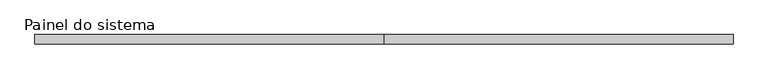
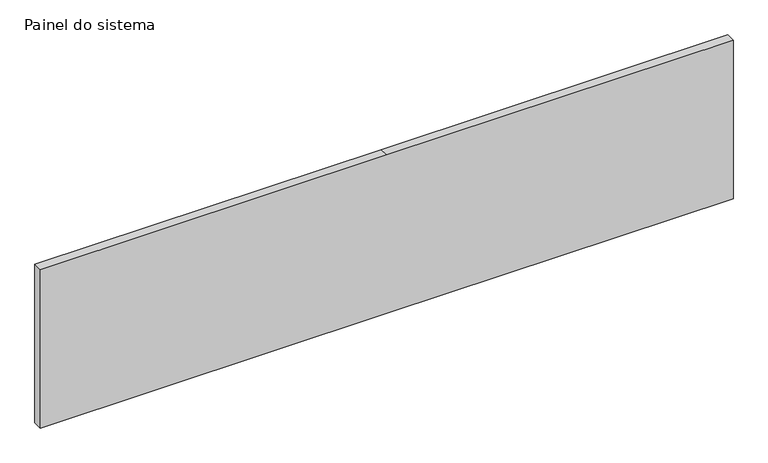
"""IFC4 building model written with IfcOpenShell, lengths in millimetres: plate geometry, Painel do sistema : Envidraçado."""

from ifc_helpers import new_model, si_unit, frame, origin, place, context, project, spatial, polyline, outline, extrude, source, transform, mapped, element, save


def painel_do_sistema_b648e332(model_context):
    return source(origin(), model_context, "Body", "SweptSolid", [
        extrude(outline(polyline([(0.0, -931.0166666), (0.0, 0.0), (0.0, 931.0166666), (450.0, 931.0166666), (450.0, 0.0), (450.0, -931.0166666), (0.0, -931.0166666)])), frame((0.0, 24.5, 0.0), z_axis=(0.0, 1.0, 0.0), x_axis=(0.0, 0.0, 1.0)), (0.0, 0.0, 1.0), 25.0),
    ])


if __name__ == "__main__":
    model = new_model("IFC4")
    model_context = context("Model", 3, world=origin())
    ifc_project = project(units=[si_unit("LENGTHUNIT", "METRE", prefix="MILLI")], contexts=[model_context])
    site = spatial("IfcSite", under=ifc_project)
    building = spatial("IfcBuilding", under=site)
    placement = place(None, origin())
    painel_do_sistema_shape = painel_do_sistema_b648e332(model_context)
    element("IfcPlate", 1, ObjectType="Painel do sistema : Envidraçado", at=placement, inside=building, context=model_context, shape_type="MappedRepresentation", body=[
        mapped(painel_do_sistema_shape, transform((0.0, 0.0, 0.0), x_axis=(1.0, 0.0, 0.0), y_axis=(0.0, 1.0, 0.0), z_axis=(0.0, 0.0, 1.0))),
    ])
    save(model, "model.ifc")

# Revit data of these elements
# Type "Painel do sistema : Envidraçado"
#   Construction Type Id = "GSP4R"
#   Analytic Construction = "Vidraça única Pilkington 1/8 pol"
#   Visual Light Transmittance = 0.9
#   Solar Heat Gain Coefficient = 0.86
#   Heat Transfer Coefficient (U) = 6.7069 W/(m²·K)
# Element 1 (IfcPlate, "Painel do sistema : Envidraçado")
#   Materials on its faces: ".VIDRO GENÉRICO"
# Materials
#   ".VIDRO GENÉRICO": class ".CC_VIDRO", colour RGB 0 128 192, transparency 0.9, Description = "Vidro comum", Cost = 0
